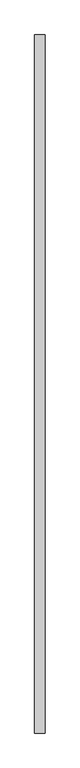
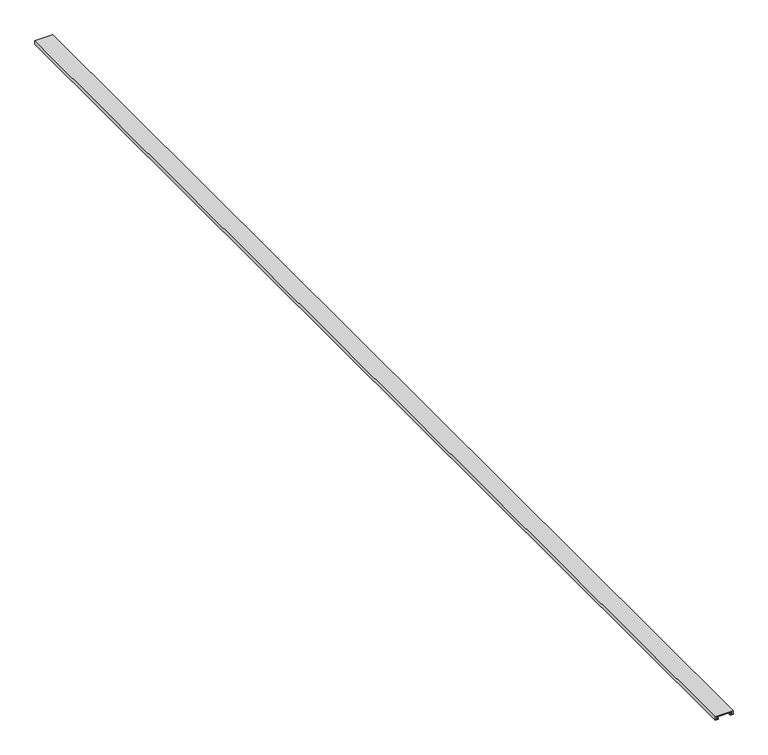
"""IFC4 building model written with IfcOpenShell, lengths in millimetres: proxy geometry, Door frame11:Door frame011:296332 : Door frame11:Door frame011:296332."""

from ifc_helpers import new_model, si_unit, frame, origin, place, context, project, spatial, polyline, outline, extrude, source, transform, mapped, element, save


def generic_models_ed7a1762(model_context):
    return source(origin(), model_context, "Body", "SweptSolid", [
        extrude(outline(polyline([(36591.6240434, 20317.2493037), (36591.6240434, 20287.0261485), (36585.6418094, 20287.0261485), (36585.6418094, 20291.9679725), (36588.2201312, 20291.9679725), (36588.2201312, 20290.9275885), (36586.9422894, 20290.9275885), (36586.9422894, 20288.3266025), (36590.0634674, 20288.3266025), (36590.0634674, 20315.9488497), (36586.9422894, 20315.9488497), (36586.9422894, 20313.5473809), (36588.2201312, 20313.5473809), (36588.2201312, 20312.3074797), (36585.6418094, 20312.3074797), (36585.6418094, 20317.2493037), (36591.6240434, 20317.2493037)])), frame((0.0, -774.5581156, 0.0), z_axis=(0.0, 1.0, 0.0), x_axis=(0.0, 0.0, 1.0)), (0.0, 0.0, 1.0), 1999.85),
    ])


if __name__ == "__main__":
    model = new_model("IFC4")
    model_context = context("Model", 3, world=origin())
    ifc_project = project(units=[si_unit("LENGTHUNIT", "METRE", prefix="MILLI")], contexts=[model_context])
    site = spatial("IfcSite", under=ifc_project)
    building = spatial("IfcBuilding", under=site)
    placement = place(None, origin())
    generic_models_shape = generic_models_ed7a1762(model_context)
    element("IfcBuildingElementProxy", 1, Name="Door frame11:Door frame011:296332 : Door frame11:Door frame011:296332", ObjectType="Door frame11:Door frame011:296332 : Door frame11:Door frame011:296332", at=placement, inside=building, context=model_context, shape_type="MappedRepresentation", body=[
        mapped(generic_models_shape, transform((0.0, 0.0, 0.0), x_axis=(1.0, 0.0, 0.0), y_axis=(0.0, 1.0, 0.0), z_axis=(0.0, 0.0, 1.0))),
    ])
    save(model, "model.ifc")

# Revit data of these elements
# Type "Door frame11:Door frame011:296332 : Door frame11:Door frame011:296332"
#   NameOverride = "Door frame11:Door frame011:296332"
#   ObjectTypeOverride = "Door frame11:Door frame011"
#   Reference = "Door frame011"
#   Category = "Generic Models"
#   Tag = "296332"
# Element 1 (IfcBuildingElementProxy, "Door frame11:Door frame011:296332 : Door frame11:Door frame011:296332")
#   Materials on its faces: "FLEETWOOD SERIES T-3200 SINGLE SWING DOOR FRAME"
# Materials
#   "FLEETWOOD SERIES T-3200 SINGLE SWING DOOR FRAME": class "Unassigned", colour RGB 128 128 128, transparency 0, Cost = 0
